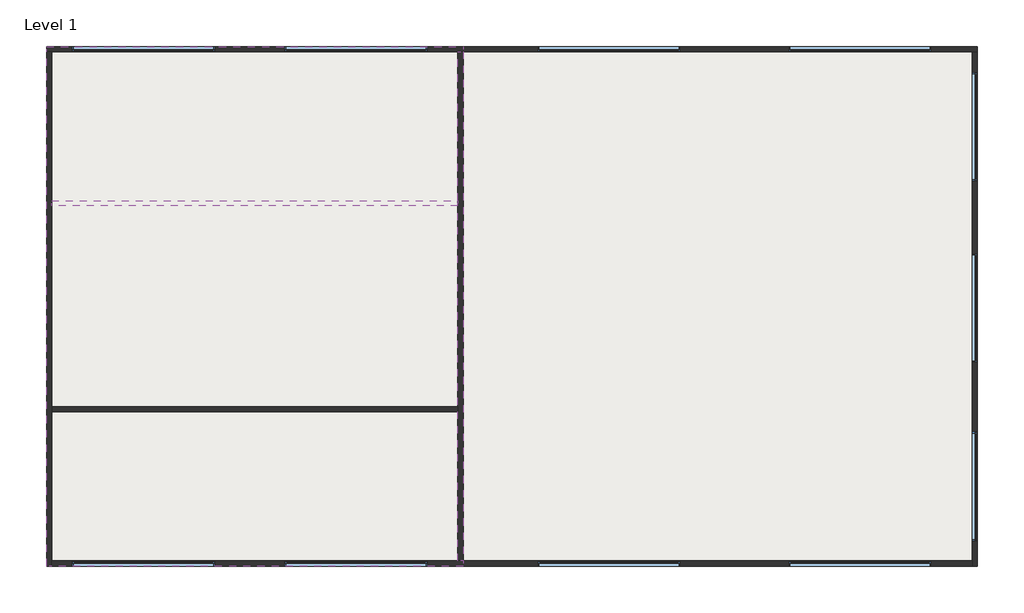
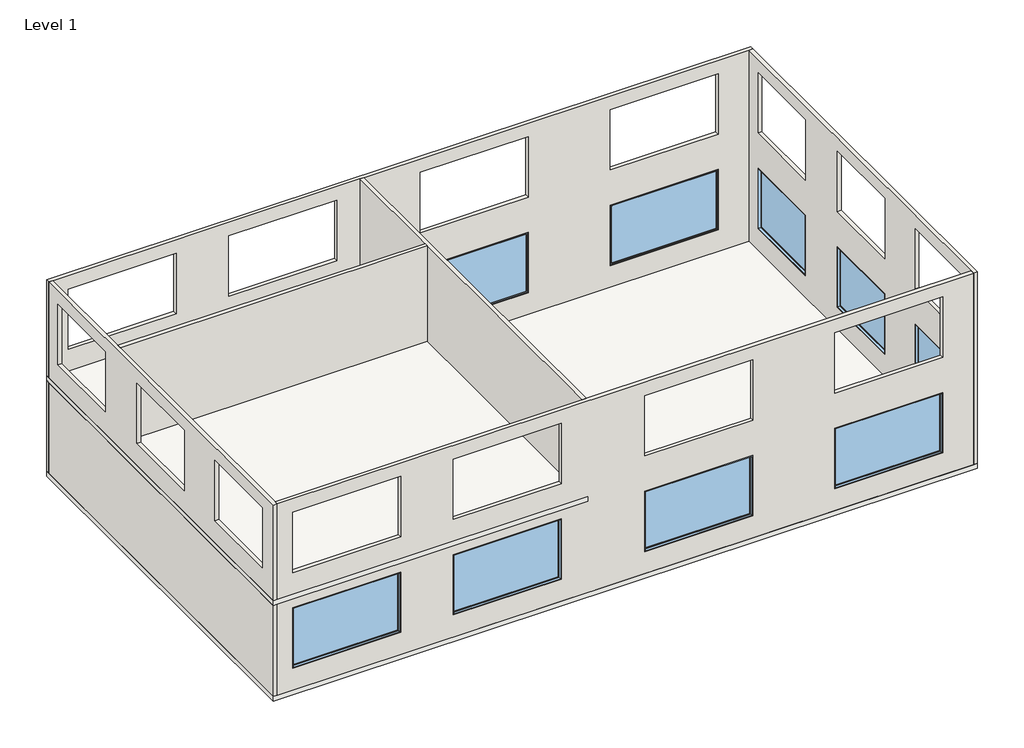
# One storey: 11 windows, 8 walls, 2 slabs.
"""IFC4 building model written with IfcOpenShell, lengths in millimetres."""

import ifcopenshell
import ifcopenshell.guid

model = None  # the IFC model being written
_history = None  # IfcOwnerHistory: only IFC2X3 demands one
_inside = {}  # id of a spatial element -> (the spatial element, [elements in it])
_under = {}  # id of a project, library or spatial element -> (it, [spatial elements below it])
_declared = {}  # id of a project -> (the project, [libraries it declares])
_typed = {}  # id of a type object -> (the type object, [elements of that type])
_made_of = {}  # id of a material, layer set ... -> (it, [elements and type objects made of it])


def new_model(schema):
    """Start an empty IFC model of exactly this schema.

    Asked for "IFC4X3", IfcOpenShell would pick the latest addendum, in which some entities
    have other attributes; the version numbers below select the first issue.
    IFC2X3 requires an IfcOwnerHistory on every rooted entity: one is made here for all.
    """
    global model, _history
    if schema == "IFC4X3":
        model = ifcopenshell.file(schema_version=(4, 3, 0, 0))
    else:
        model = ifcopenshell.file(schema=schema)
    _inside.clear()
    _under.clear()
    _declared.clear()
    _typed.clear()
    _made_of.clear()
    _history = None
    if model.schema == "IFC2X3":
        org = make("IfcOrganization", Name="unknown")
        user = make(
            "IfcPersonAndOrganization",
            ThePerson=make("IfcPerson", FamilyName="unknown"),
            TheOrganization=org,
        )
        app = make(
            "IfcApplication",
            ApplicationDeveloper=org,
            Version="unknown",
            ApplicationFullName="unknown",
            ApplicationIdentifier="unknown",
        )
        _history = make(
            "IfcOwnerHistory",
            OwningUser=user,
            OwningApplication=app,
            ChangeAction="ADDED",
            CreationDate=0,
        )
    return model


def make(cls, **values):
    """One entity of the class cls with the attributes given. An attribute that is None is left unset."""
    return model.create_entity(
        cls, **{name: value for name, value in values.items() if value is not None}
    )


def rooted(cls, **values):
    """An entity with a GlobalId (a new one), such as an element, a storey or a relation."""
    return make(cls, GlobalId=ifcopenshell.guid.new(), OwnerHistory=_history, **values)


def si_unit(unit_type, name, prefix=None):
    """IfcSIUnit, for example si_unit("LENGTHUNIT", "METRE", prefix="MILLI")."""
    return make("IfcSIUnit", UnitType=unit_type, Prefix=prefix, Name=name)


def assignment(units):
    """IfcUnitAssignment: the units of a project."""
    return None if units is None else make("IfcUnitAssignment", Units=units)


def point(xyz):
    """IfcCartesianPoint."""
    return None if xyz is None else make("IfcCartesianPoint", Coordinates=xyz)


def direction(xyz):
    """IfcDirection."""
    return None if xyz is None else make("IfcDirection", DirectionRatios=xyz)


def frame(location, z_axis=None, x_axis=None):
    """IfcAxis2Placement3D, a coordinate frame: its origin and axes. An axis left out is left unset."""
    return make(
        "IfcAxis2Placement3D",
        Location=point(location),
        Axis=direction(z_axis),
        RefDirection=direction(x_axis),
    )


def origin():
    """The frame at (0, 0, 0) with its axes left unset."""
    return frame((0.0, 0.0, 0.0))


def origin_with_axes():
    """The frame at (0, 0, 0) with the z axis (0, 0, 1) and the x axis (1, 0, 0) written out."""
    return frame((0.0, 0.0, 0.0), z_axis=(0.0, 0.0, 1.0), x_axis=(1.0, 0.0, 0.0))


def place(relative_to, where):
    """IfcLocalPlacement: puts the frame where relative to a parent placement (None: the world)."""
    return make(
        "IfcLocalPlacement", PlacementRelTo=relative_to, RelativePlacement=where
    )


def context(
    kind, dimensions, precision=None, world=None, true_north=None, identifier=None
):
    """IfcGeometricRepresentationContext, for example the 3D "Model" context."""
    return make(
        "IfcGeometricRepresentationContext",
        ContextIdentifier=identifier,
        ContextType=kind,
        CoordinateSpaceDimension=dimensions,
        Precision=precision,
        WorldCoordinateSystem=world,
        TrueNorth=true_north,
    )


def project(units=None, contexts=None):
    """IfcProject with its units and contexts."""
    return rooted(
        "IfcProject",
        Name="project",
        RepresentationContexts=contexts,
        UnitsInContext=assignment(units),
    )


def spatial(cls, under=None, at=None, **own):
    """A site, building, storey or space (cls), placed at a placement, below another one or the project."""
    s = rooted(cls, ObjectPlacement=at, **own)
    if under is not None:
        _under.setdefault(under.id(), (under, []))[1].append(s)
    return s


def polyline(points):
    """IfcPolyline through the points."""
    return make("IfcPolyline", Points=[point(p) for p in points])


def outline(outer, holes=None, kind="AREA"):
    """IfcArbitraryClosedProfileDef: a profile drawn as a closed curve; with holes, ...WithVoids."""
    if holes is None:
        return make("IfcArbitraryClosedProfileDef", ProfileType=kind, OuterCurve=outer)
    return make(
        "IfcArbitraryProfileDefWithVoids",
        ProfileType=kind,
        OuterCurve=outer,
        InnerCurves=holes,
    )


def extrude(swept, where, along, depth):
    """IfcExtrudedAreaSolid: the profile swept, set in the frame where, extruded along a direction by depth."""
    return make(
        "IfcExtrudedAreaSolid",
        SweptArea=swept,
        Position=where,
        ExtrudedDirection=direction(along),
        Depth=depth,
    )


def faces_of(points, faces, orient=None, outer=None):
    """IfcFace entities. A face is a list of loops; a loop is a list of indices into points, from 0.

    orient and outer hold one flag for each loop. By default every Orientation is true, the
    first loop of a face is its IfcFaceOuterBound and the others are IfcFaceBound.
    """
    made = []
    for i, loops in enumerate(faces):
        bounds = []
        for j, loop in enumerate(loops):
            is_outer = j == 0 if outer is None else outer[i][j]
            bounds.append(
                make(
                    "IfcFaceOuterBound" if is_outer else "IfcFaceBound",
                    Bound=make("IfcPolyLoop", Polygon=[points[k] for k in loop]),
                    Orientation=True if orient is None else orient[i][j],
                )
            )
        made.append(make("IfcFace", Bounds=bounds))
    return made


def faceted_brep(points, faces, orient=None, outer=None, voids=None):
    """IfcFacetedBrep: a solid bounded by flat faces; with voids (closed shells), ...WithVoids."""
    shared = [point(p) for p in points]
    hull = make("IfcClosedShell", CfsFaces=faces_of(shared, faces, orient, outer))
    if voids is None:
        return make("IfcFacetedBrep", Outer=hull)
    return make(
        "IfcFacetedBrepWithVoids",
        Outer=hull,
        Voids=[
            make(cls, CfsFaces=faces_of(shared, fs, o, b)) for cls, fs, o, b in voids
        ],
    )


def shape(context_of_items, identifier, shape_type, items):
    """IfcShapeRepresentation: the items that make up one representation, for example the "Body"."""
    return make(
        "IfcShapeRepresentation",
        ContextOfItems=context_of_items,
        RepresentationIdentifier=identifier,
        RepresentationType=shape_type,
        Items=items,
    )


def source(mapping_origin, context_of_items, identifier, shape_type, items):
    """IfcRepresentationMap: a shape defined once, which mapped items show again and again."""
    return make(
        "IfcRepresentationMap",
        MappingOrigin=mapping_origin,
        MappedRepresentation=shape(context_of_items, identifier, shape_type, items),
    )


def transform(
    local_origin,
    x_axis=None,
    y_axis=None,
    z_axis=None,
    scale=None,
    scale2=None,
    scale3=None,
    uniform=True,
):
    """IfcCartesianTransformationOperator3D, or its non-uniform kind. x_axis, y_axis, z_axis: its Axis1, 2, 3."""
    if uniform:
        return make(
            "IfcCartesianTransformationOperator3D",
            Axis1=direction(x_axis),
            Axis2=direction(y_axis),
            LocalOrigin=point(local_origin),
            Scale=scale,
            Axis3=direction(z_axis),
        )
    return make(
        "IfcCartesianTransformationOperator3DnonUniform",
        Axis1=direction(x_axis),
        Axis2=direction(y_axis),
        LocalOrigin=point(local_origin),
        Scale=scale,
        Axis3=direction(z_axis),
        Scale2=scale2,
        Scale3=scale3,
    )


def mapped(mapping_source, mapping_target):
    """IfcMappedItem: shows the shape of a source again, moved by a transform."""
    return make(
        "IfcMappedItem", MappingSource=mapping_source, MappingTarget=mapping_target
    )


def made_of(thing, what):
    """Note that an element or type object is made of a material, layer set ...; save() writes the relation."""
    if what is not None:
        _made_of.setdefault(what.id(), (what, []))[1].append(thing)
    return thing


def element(
    cls,
    number,
    at=None,
    inside=None,
    cuts=None,
    type_object=None,
    material=None,
    context=None,
    identifier="Body",
    shape_type=None,
    held_by="IfcProductDefinitionShape",
    body=None,
    shapes=None,
    **own,
):
    """One element of the class cls, such as IfcWall. Its Tag is "e" and its number.

    at: its placement. inside: the storey or other place that contains it. cuts: it is an
    opening in that element (IfcRelVoidsElement). A single representation is given by context,
    identifier, shape_type and body (its items); several are given by shapes. held_by: the class
    of the entity that holds the representations. save() writes the other relations.
    """
    e = rooted(cls, Tag="e%d" % number, ObjectPlacement=at, **own)
    if body is not None:
        shapes = [shape(context, identifier, shape_type, body)]
    if shapes is not None:
        e.Representation = make(held_by, Representations=shapes)
    if inside is not None:
        _inside.setdefault(inside.id(), (inside, []))[1].append(e)
    if cuts is not None:
        rooted(
            "IfcRelVoidsElement", RelatingBuildingElement=cuts, RelatedOpeningElement=e
        )
    if type_object is not None:
        _typed.setdefault(type_object.id(), (type_object, []))[1].append(e)
    return made_of(e, material)


def aggregate(whole, parts):
    """IfcRelAggregates: a whole, such as a stair, and the parts it consists of."""
    return rooted("IfcRelAggregates", RelatingObject=whole, RelatedObjects=parts)


def save(model, path):
    """Write the relations noted so far, then the file.

    IfcRelAggregates (storeys below a building ...), IfcRelContainedInSpatialStructure (elements
    in a storey), IfcRelDefinesByType, IfcRelAssociatesMaterial and IfcRelDeclares: one each for
    every whole, place, type object, material and project.
    """
    for whole, parts in _under.values():
        aggregate(whole, parts)
    for where, things in _inside.values():
        rooted(
            "IfcRelContainedInSpatialStructure",
            RelatedElements=things,
            RelatingStructure=where,
        )
    for kind, things in _typed.values():
        rooted("IfcRelDefinesByType", RelatedObjects=things, RelatingType=kind)
    for what, things in _made_of.values():
        rooted("IfcRelAssociatesMaterial", RelatedObjects=things, RelatingMaterial=what)
    for by, libraries in _declared.values():
        rooted("IfcRelDeclares", RelatingContext=by, RelatedDefinitions=libraries)
    model.write(path)


def m_fixed_2500x_4228mm_fd5e51e7(model_context):
    return source(origin(), model_context, "Body", "SweptSolid", [
        extrude(outline(polyline([(-2050.8, 54.2), (2050.8, 54.2), (2050.8, 42.2), (-2050.8, 42.2), (-2050.8, 54.2)])), frame((0.0, 0.0, 368.0), z_axis=(0.0, 0.0, 1.0), x_axis=(1.0, 0.0, 0.0)), (0.0, 0.0, 1.0), 2374.0),
        extrude(outline(polyline([(2786.0, -2094.8), (324.0, -2094.8), (324.0, 2094.8), (2786.0, 2094.8), (2786.0, -2094.8)]), holes=[polyline([(2742.0, -2050.8), (2742.0, 2050.8), (368.0, 2050.8), (368.0, -2050.8), (2742.0, -2050.8)])]), frame((0.0, 26.2, 0.0), z_axis=(0.0, 1.0, 0.0), x_axis=(0.0, 0.0, 1.0)), (0.0, 0.0, 1.0), 44.0),
        extrude(outline(polyline([(2805.0, -2113.8), (305.0, -2113.8), (305.0, 2113.8), (2805.0, 2113.8), (2805.0, -2113.8)]), holes=[polyline([(2786.0, -2094.8), (2786.0, 2094.8), (324.0, 2094.8), (324.0, -2094.8), (2786.0, -2094.8)])]), frame((0.0, 26.2, 0.0), z_axis=(0.0, 1.0, 0.0), x_axis=(0.0, 0.0, 1.0)), (0.0, 0.0, 1.0), 63.0),
        extrude(outline(polyline([(2805.0, -2113.8), (305.0, -2113.8), (305.0, 2113.8), (2805.0, 2113.8), (2805.0, -2113.8)]), holes=[polyline([(2773.0, -2081.8), (2773.0, 2081.8), (337.0, 2081.8), (337.0, -2081.8), (2773.0, -2081.8)])]), frame((0.0, -63.2, 0.0), z_axis=(0.0, 1.0, 0.0), x_axis=(0.0, 0.0, 1.0)), (0.0, 0.0, 1.0), 89.4),
    ])


def m_fixed_2500x_4228mm_f14c179f(model_context):
    return source(origin(), model_context, "Body", "SweptSolid", [
        extrude(outline(polyline([(-2050.8, -54.2), (-2050.8, -42.2), (2050.8, -42.2), (2050.8, -54.2), (-2050.8, -54.2)])), frame((0.0, 0.0, 368.0), z_axis=(0.0, 0.0, 1.0), x_axis=(1.0, 0.0, 0.0)), (0.0, 0.0, 1.0), 2374.0),
        extrude(outline(polyline([(2786.0, -2094.8), (324.0, -2094.8), (324.0, 2094.8), (2786.0, 2094.8), (2786.0, -2094.8)]), holes=[polyline([(2742.0, -2050.8), (2742.0, 2050.8), (368.0, 2050.8), (368.0, -2050.8), (2742.0, -2050.8)])]), frame((0.0, -70.2, 0.0), z_axis=(0.0, 1.0, 0.0), x_axis=(0.0, 0.0, 1.0)), (0.0, 0.0, 1.0), 44.0),
        extrude(outline(polyline([(2805.0, -2113.8), (305.0, -2113.8), (305.0, 2113.8), (2805.0, 2113.8), (2805.0, -2113.8)]), holes=[polyline([(2786.0, -2094.8), (2786.0, 2094.8), (324.0, 2094.8), (324.0, -2094.8), (2786.0, -2094.8)])]), frame((0.0, -89.2, 0.0), z_axis=(0.0, 1.0, 0.0), x_axis=(0.0, 0.0, 1.0)), (0.0, 0.0, 1.0), 63.0),
        extrude(outline(polyline([(2805.0, -2113.8), (305.0, -2113.8), (305.0, 2113.8), (2805.0, 2113.8), (2805.0, -2113.8)]), holes=[polyline([(2773.0, -2081.8), (2773.0, 2081.8), (337.0, 2081.8), (337.0, -2081.8), (2773.0, -2081.8)])]), frame((0.0, -26.2, 0.0), z_axis=(0.0, 1.0, 0.0), x_axis=(0.0, 0.0, 1.0)), (0.0, 0.0, 1.0), 89.4),
    ])


def m_fixed_2500x_3220mm_8b997f8c(model_context):
    return source(origin(), model_context, "Body", "SweptSolid", [
        extrude(outline(polyline([(-1546.8, -54.2), (-1546.8, -42.2), (1546.8, -42.2), (1546.8, -54.2), (-1546.8, -54.2)])), frame((0.0, 0.0, 368.0), z_axis=(0.0, 0.0, 1.0), x_axis=(1.0, 0.0, 0.0)), (0.0, 0.0, 1.0), 2374.0),
        extrude(outline(polyline([(2786.0, -1590.8), (324.0, -1590.8), (324.0, 1590.8), (2786.0, 1590.8), (2786.0, -1590.8)]), holes=[polyline([(2742.0, -1546.8), (2742.0, 1546.8), (368.0, 1546.8), (368.0, -1546.8), (2742.0, -1546.8)])]), frame((0.0, -70.2, 0.0), z_axis=(0.0, 1.0, 0.0), x_axis=(0.0, 0.0, 1.0)), (0.0, 0.0, 1.0), 44.0),
        extrude(outline(polyline([(2805.0, -1609.8), (305.0, -1609.8), (305.0, 1609.8), (2805.0, 1609.8), (2805.0, -1609.8)]), holes=[polyline([(2786.0, -1590.8), (2786.0, 1590.8), (324.0, 1590.8), (324.0, -1590.8), (2786.0, -1590.8)])]), frame((0.0, -89.2, 0.0), z_axis=(0.0, 1.0, 0.0), x_axis=(0.0, 0.0, 1.0)), (0.0, 0.0, 1.0), 63.0),
        extrude(outline(polyline([(2805.0, -1609.8), (305.0, -1609.8), (305.0, 1609.8), (2805.0, 1609.8), (2805.0, -1609.8)]), holes=[polyline([(2773.0, -1577.8), (2773.0, 1577.8), (337.0, 1577.8), (337.0, -1577.8), (2773.0, -1577.8)])]), frame((0.0, -26.2, 0.0), z_axis=(0.0, 1.0, 0.0), x_axis=(0.0, 0.0, 1.0)), (0.0, 0.0, 1.0), 89.4),
    ])


model = new_model("IFC4")

# Units and contexts
model_context = context("Model", 3, world=origin())
ifc_project = project(units=[si_unit("LENGTHUNIT", "METRE", prefix="MILLI")], contexts=[model_context])

# Site, building, storey
site = spatial("IfcSite", under=ifc_project)
building = spatial("IfcBuilding", under=site)
storey = spatial("IfcBuildingStorey", under=building, Name="Level 1", Elevation=0.0)

# Slabs
placement = place(None, origin())
element("IfcSlab", 1, ObjectType="160mm Concrete With 50mm Metal Deck", at=placement, inside=storey, context=model_context, shape_type="Brep", body=[
    faceted_brep([(29068.464681, 11296.9802217, -210.0), (29068.464681, -4095.4197783, -210.0), (1484.064681, -4095.4197783, -210.0), (1484.064681, 11296.9802217, -210.0), (29068.464681, 11296.9802217, 0.0), (1484.064681, 11296.9802217, 0.0), (1484.064681, -4095.4197783, 0.0), (28916.064681, -4095.4197783, 0.0), (29068.464681, -4095.4197783, 0.0), (29068.464681, 11144.5802217, 0.0)], [[[0, 1, 2, 3]], [[4, 5, 6, 7, 8, 9]], [[1, 0, 4, 9, 8]], [[2, 1, 8, 7, 6]], [[3, 2, 6, 5]], [[0, 3, 5, 4]]]),
])
element("IfcSlab", 2, ObjectType="160mm Concrete With 50mm Metal Deck", at=placement, inside=storey, context=model_context, shape_type="Brep", body=[
    faceted_brep([(13828.464681, 11296.9802217, 3752.4), (13828.464681, 11144.5802217, 3752.4), (13828.464681, -3943.0197783, 3752.4), (13828.464681, -4095.4197783, 3752.4), (1636.464681, -4095.4197783, 3752.4), (1484.064681, -4095.4197783, 3752.4), (1484.064681, 11144.5802217, 3752.4), (1484.064681, 11296.9802217, 3752.4), (13828.464681, 11296.9802217, 3962.4), (1484.064681, 11296.9802217, 3962.4), (1484.064681, 11144.5802217, 3962.4), (1484.064681, -4095.4197783, 3962.4), (1636.464681, -4095.4197783, 3962.4), (13828.464681, -4095.4197783, 3962.4), (13828.464681, -3943.0197783, 3962.4), (13828.464681, 11144.5802217, 3962.4)], [[[0, 1, 2, 3, 4, 5, 6, 7]], [[8, 9, 10, 11, 12, 13, 14, 15]], [[3, 2, 1, 0, 8, 15, 14, 13]], [[5, 4, 3, 13, 12, 11]], [[7, 6, 5, 11, 10, 9]], [[0, 7, 9, 8]]]),
])

# Walls
element("IfcWall", 3, ObjectType="Generic - 152.4mm", at=placement, inside=storey, context=model_context, shape_type="Brep", body=[
    faceted_brep([(1484.064681, 11144.5802217, 0.0), (1636.464681, 11144.5802217, 0.0), (13676.064681, 11144.5802217, 0.0), (13828.464681, 11144.5802217, 0.0), (28916.064681, 11144.5802217, 0.0), (29068.464681, 11144.5802217, 0.0), (29068.464681, 11144.5802217, 7924.8), (28916.064681, 11144.5802217, 7924.8), (13828.464681, 11144.5802217, 7924.8), (13676.064681, 11144.5802217, 7924.8), (1636.464681, 11144.5802217, 7924.8), (1484.064681, 11144.5802217, 7924.8), (1484.064681, 11144.5802217, 3962.4), (13676.064681, 11144.5802217, 3962.4), (13828.464681, 11144.5802217, 3962.4), (13828.464681, 11144.5802217, 3752.4), (13676.064681, 11144.5802217, 3752.4), (1484.064681, 11144.5802217, 3752.4), (6474.064681, 11144.5802217, 3402.4), (6474.064681, 11144.5802217, 902.4), (2246.464681, 11144.5802217, 902.4), (2246.464681, 11144.5802217, 3402.4), (12766.064681, 11144.5802217, 3402.4), (12766.064681, 11144.5802217, 902.4), (8538.464681, 11144.5802217, 902.4), (8538.464681, 11144.5802217, 3402.4), (20266.064681, 11144.5802217, 3402.4), (20266.064681, 11144.5802217, 902.4), (16038.464681, 11144.5802217, 902.4), (16038.464681, 11144.5802217, 3402.4), (27706.064681, 11144.5802217, 3402.4), (27706.064681, 11144.5802217, 902.4), (23478.464681, 11144.5802217, 902.4), (23478.464681, 11144.5802217, 3402.4), (27706.064681, 11144.5802217, 7362.4), (27706.064681, 11144.5802217, 4862.4), (23478.464681, 11144.5802217, 4862.4), (23478.464681, 11144.5802217, 7362.4), (20266.064681, 11144.5802217, 7362.4), (20266.064681, 11144.5802217, 4862.4), (16038.464681, 11144.5802217, 4862.4), (16038.464681, 11144.5802217, 7362.4), (12766.064681, 11144.5802217, 7362.4), (12766.064681, 11144.5802217, 4862.4), (8538.464681, 11144.5802217, 4862.4), (8538.464681, 11144.5802217, 7362.4), (6474.064681, 11144.5802217, 7362.4), (6474.064681, 11144.5802217, 4862.4), (2246.464681, 11144.5802217, 4862.4), (2246.464681, 11144.5802217, 7362.4), (29068.464681, 11296.9802217, 0.0), (1484.064681, 11296.9802217, 0.0), (1484.064681, 11296.9802217, 3752.4), (13828.464681, 11296.9802217, 3752.4), (13828.464681, 11296.9802217, 3962.4), (1484.064681, 11296.9802217, 3962.4), (1484.064681, 11296.9802217, 7924.8), (29068.464681, 11296.9802217, 7924.8), (6474.064681, 11296.9802217, 902.4), (6474.064681, 11296.9802217, 3402.4), (2246.464681, 11296.9802217, 3402.4), (2246.464681, 11296.9802217, 902.4), (12766.064681, 11296.9802217, 902.4), (12766.064681, 11296.9802217, 3402.4), (8538.464681, 11296.9802217, 3402.4), (8538.464681, 11296.9802217, 902.4), (20266.064681, 11296.9802217, 902.4), (20266.064681, 11296.9802217, 3402.4), (16038.464681, 11296.9802217, 3402.4), (16038.464681, 11296.9802217, 902.4), (27706.064681, 11296.9802217, 902.4), (27706.064681, 11296.9802217, 3402.4), (23478.464681, 11296.9802217, 3402.4), (23478.464681, 11296.9802217, 902.4), (27706.064681, 11296.9802217, 4862.4), (27706.064681, 11296.9802217, 7362.4), (23478.464681, 11296.9802217, 7362.4), (23478.464681, 11296.9802217, 4862.4), (20266.064681, 11296.9802217, 4862.4), (20266.064681, 11296.9802217, 7362.4), (16038.464681, 11296.9802217, 7362.4), (16038.464681, 11296.9802217, 4862.4), (12766.064681, 11296.9802217, 4862.4), (12766.064681, 11296.9802217, 7362.4), (8538.464681, 11296.9802217, 7362.4), (8538.464681, 11296.9802217, 4862.4), (6474.064681, 11296.9802217, 4862.4), (6474.064681, 11296.9802217, 7362.4), (2246.464681, 11296.9802217, 7362.4), (2246.464681, 11296.9802217, 4862.4)], [[[0, 1, 2, 3, 4, 5, 6, 7, 8, 9, 10, 11, 12, 13, 14, 15, 16, 17], [18, 19, 20, 21], [22, 23, 24, 25], [26, 27, 28, 29], [30, 31, 32, 33], [34, 35, 36, 37], [38, 39, 40, 41], [42, 43, 44, 45], [46, 47, 48, 49]], [[50, 51, 52, 53, 54, 55, 56, 57], [58, 59, 60, 61], [62, 63, 64, 65], [66, 67, 68, 69], [70, 71, 72, 73], [74, 75, 76, 77], [78, 79, 80, 81], [82, 83, 84, 85], [86, 87, 88, 89]], [[5, 4, 3, 2, 1, 0, 51, 50]], [[11, 10, 9, 8, 7, 6, 57, 56]], [[6, 5, 50, 57]], [[11, 56, 55, 12]], [[51, 0, 17, 52]], [[59, 58, 19, 18]], [[60, 59, 18, 21]], [[61, 60, 21, 20]], [[58, 61, 20, 19]], [[63, 62, 23, 22]], [[64, 63, 22, 25]], [[65, 64, 25, 24]], [[62, 65, 24, 23]], [[67, 66, 27, 26]], [[68, 67, 26, 29]], [[69, 68, 29, 28]], [[66, 69, 28, 27]], [[71, 70, 31, 30]], [[72, 71, 30, 33]], [[73, 72, 33, 32]], [[70, 73, 32, 31]], [[75, 74, 35, 34]], [[76, 75, 34, 37]], [[77, 76, 37, 36]], [[74, 77, 36, 35]], [[79, 78, 39, 38]], [[80, 79, 38, 41]], [[81, 80, 41, 40]], [[78, 81, 40, 39]], [[83, 82, 43, 42]], [[84, 83, 42, 45]], [[85, 84, 45, 44]], [[82, 85, 44, 43]], [[87, 86, 47, 46]], [[88, 87, 46, 49]], [[89, 88, 49, 48]], [[86, 89, 48, 47]], [[15, 53, 52, 17, 16]], [[54, 14, 13, 12, 55]], [[53, 15, 14, 54]]]),
])
element("IfcWall", 4, ObjectType="Generic - 152.4mm", at=placement, inside=storey, context=model_context, shape_type="Brep", body=[
    faceted_brep([(28916.064681, 11144.5802217, 0.0), (28916.064681, -3943.0197783, 0.0), (28916.064681, -4095.4197783, 0.0), (28916.064681, -4095.4197783, 7924.8), (28916.064681, -3943.0197783, 7924.8), (28916.064681, 11144.5802217, 7924.8), (28916.064681, -3343.0197783, 902.4), (28916.064681, -123.4197783, 902.4), (28916.064681, -123.4197783, 3402.4), (28916.064681, -3343.0197783, 3402.4), (28916.064681, 1942.9802217, 902.4), (28916.064681, 5162.5802217, 902.4), (28916.064681, 5162.5802217, 3402.4), (28916.064681, 1942.9802217, 3402.4), (28916.064681, 7310.9802217, 902.4), (28916.064681, 10530.5802217, 902.4), (28916.064681, 10530.5802217, 3402.4), (28916.064681, 7310.9802217, 3402.4), (28916.064681, -3343.0197783, 4864.8), (28916.064681, -123.4197783, 4864.8), (28916.064681, -123.4197783, 7364.8), (28916.064681, -3343.0197783, 7364.8), (28916.064681, 1942.9802217, 4864.8), (28916.064681, 5162.5802217, 4864.8), (28916.064681, 5162.5802217, 7364.8), (28916.064681, 1942.9802217, 7364.8), (28916.064681, 7310.9802217, 4864.8), (28916.064681, 10530.5802217, 4864.8), (28916.064681, 10530.5802217, 7364.8), (28916.064681, 7310.9802217, 7364.8), (29068.464681, 11144.5802217, 0.0), (29068.464681, 11144.5802217, 7924.8), (29068.464681, -4095.4197783, 7924.8), (29068.464681, -4095.4197783, 0.0), (29068.464681, -3343.0197783, 902.4), (29068.464681, -3343.0197783, 3402.4), (29068.464681, -123.4197783, 3402.4), (29068.464681, -123.4197783, 902.4), (29068.464681, 1942.9802217, 902.4), (29068.464681, 1942.9802217, 3402.4), (29068.464681, 5162.5802217, 3402.4), (29068.464681, 5162.5802217, 902.4), (29068.464681, 7310.9802217, 902.4), (29068.464681, 7310.9802217, 3402.4), (29068.464681, 10530.5802217, 3402.4), (29068.464681, 10530.5802217, 902.4), (29068.464681, -3343.0197783, 4864.8), (29068.464681, -3343.0197783, 7364.8), (29068.464681, -123.4197783, 7364.8), (29068.464681, -123.4197783, 4864.8), (29068.464681, 1942.9802217, 4864.8), (29068.464681, 1942.9802217, 7364.8), (29068.464681, 5162.5802217, 7364.8), (29068.464681, 5162.5802217, 4864.8), (29068.464681, 7310.9802217, 4864.8), (29068.464681, 7310.9802217, 7364.8), (29068.464681, 10530.5802217, 7364.8), (29068.464681, 10530.5802217, 4864.8)], [[[0, 1, 2, 3, 4, 5], [6, 7, 8, 9], [10, 11, 12, 13], [14, 15, 16, 17], [18, 19, 20, 21], [22, 23, 24, 25], [26, 27, 28, 29]], [[30, 31, 32, 33], [34, 35, 36, 37], [38, 39, 40, 41], [42, 43, 44, 45], [46, 47, 48, 49], [50, 51, 52, 53], [54, 55, 56, 57]], [[2, 1, 0, 30, 33]], [[5, 4, 3, 32, 31]], [[0, 5, 31, 30]], [[35, 34, 6, 9]], [[36, 35, 9, 8]], [[37, 36, 8, 7]], [[34, 37, 7, 6]], [[39, 38, 10, 13]], [[40, 39, 13, 12]], [[41, 40, 12, 11]], [[38, 41, 11, 10]], [[43, 42, 14, 17]], [[44, 43, 17, 16]], [[45, 44, 16, 15]], [[42, 45, 15, 14]], [[3, 2, 33, 32]], [[47, 46, 18, 21]], [[48, 47, 21, 20]], [[49, 48, 20, 19]], [[46, 49, 19, 18]], [[51, 50, 22, 25]], [[52, 51, 25, 24]], [[53, 52, 24, 23]], [[50, 53, 23, 22]], [[55, 54, 26, 29]], [[56, 55, 29, 28]], [[57, 56, 28, 27]], [[54, 57, 27, 26]]]),
])
element("IfcWall", 5, ObjectType="Generic - 152.4mm", at=placement, inside=storey, context=model_context, shape_type="Brep", body=[
    faceted_brep([(28916.064681, -3943.0197783, 0.0), (13828.464681, -3943.0197783, 0.0), (13676.064681, -3943.0197783, 0.0), (1636.464681, -3943.0197783, 0.0), (1636.464681, -3943.0197783, 3752.4), (13676.064681, -3943.0197783, 3752.4), (13828.464681, -3943.0197783, 3752.4), (13828.464681, -3943.0197783, 3962.4), (13676.064681, -3943.0197783, 3962.4), (1636.464681, -3943.0197783, 3962.4), (1636.464681, -3943.0197783, 7924.8), (13676.064681, -3943.0197783, 7924.8), (13828.464681, -3943.0197783, 7924.8), (28916.064681, -3943.0197783, 7924.8), (27706.064681, -3943.0197783, 902.4), (27706.064681, -3943.0197783, 3402.4), (23478.464681, -3943.0197783, 3402.4), (23478.464681, -3943.0197783, 902.4), (20266.064681, -3943.0197783, 902.4), (20266.064681, -3943.0197783, 3402.4), (16038.464681, -3943.0197783, 3402.4), (16038.464681, -3943.0197783, 902.4), (12766.064681, -3943.0197783, 902.4), (12766.064681, -3943.0197783, 3402.4), (8538.464681, -3943.0197783, 3402.4), (8538.464681, -3943.0197783, 902.4), (6474.064681, -3943.0197783, 902.4), (6474.064681, -3943.0197783, 3402.4), (2246.464681, -3943.0197783, 3402.4), (2246.464681, -3943.0197783, 902.4), (27706.064681, -3943.0197783, 4862.4), (27706.064681, -3943.0197783, 7362.4), (23478.464681, -3943.0197783, 7362.4), (23478.464681, -3943.0197783, 4862.4), (20266.064681, -3943.0197783, 4862.4), (20266.064681, -3943.0197783, 7362.4), (16038.464681, -3943.0197783, 7362.4), (16038.464681, -3943.0197783, 4862.4), (12766.064681, -3943.0197783, 4862.4), (12766.064681, -3943.0197783, 7362.4), (8538.464681, -3943.0197783, 7362.4), (8538.464681, -3943.0197783, 4862.4), (6474.064681, -3943.0197783, 4862.4), (6474.064681, -3943.0197783, 7362.4), (2246.464681, -3943.0197783, 7362.4), (2246.464681, -3943.0197783, 4862.4), (1636.464681, -4095.4197783, 0.0), (28916.064681, -4095.4197783, 0.0), (28916.064681, -4095.4197783, 7924.8), (1636.464681, -4095.4197783, 7924.8), (1636.464681, -4095.4197783, 3962.4), (13828.464681, -4095.4197783, 3962.4), (13828.464681, -4095.4197783, 3752.4), (1636.464681, -4095.4197783, 3752.4), (27706.064681, -4095.4197783, 3402.4), (27706.064681, -4095.4197783, 902.4), (23478.464681, -4095.4197783, 902.4), (23478.464681, -4095.4197783, 3402.4), (20266.064681, -4095.4197783, 3402.4), (20266.064681, -4095.4197783, 902.4), (16038.464681, -4095.4197783, 902.4), (16038.464681, -4095.4197783, 3402.4), (12766.064681, -4095.4197783, 3402.4), (12766.064681, -4095.4197783, 902.4), (8538.464681, -4095.4197783, 902.4), (8538.464681, -4095.4197783, 3402.4), (6474.064681, -4095.4197783, 3402.4), (6474.064681, -4095.4197783, 902.4), (2246.464681, -4095.4197783, 902.4), (2246.464681, -4095.4197783, 3402.4), (27706.064681, -4095.4197783, 7362.4), (27706.064681, -4095.4197783, 4862.4), (23478.464681, -4095.4197783, 4862.4), (23478.464681, -4095.4197783, 7362.4), (20266.064681, -4095.4197783, 7362.4), (20266.064681, -4095.4197783, 4862.4), (16038.464681, -4095.4197783, 4862.4), (16038.464681, -4095.4197783, 7362.4), (12766.064681, -4095.4197783, 7362.4), (12766.064681, -4095.4197783, 4862.4), (8538.464681, -4095.4197783, 4862.4), (8538.464681, -4095.4197783, 7362.4), (6474.064681, -4095.4197783, 7362.4), (6474.064681, -4095.4197783, 4862.4), (2246.464681, -4095.4197783, 4862.4), (2246.464681, -4095.4197783, 7362.4)], [[[0, 1, 2, 3, 4, 5, 6, 7, 8, 9, 10, 11, 12, 13], [14, 15, 16, 17], [18, 19, 20, 21], [22, 23, 24, 25], [26, 27, 28, 29], [30, 31, 32, 33], [34, 35, 36, 37], [38, 39, 40, 41], [42, 43, 44, 45]], [[46, 47, 48, 49, 50, 51, 52, 53], [54, 55, 56, 57], [58, 59, 60, 61], [62, 63, 64, 65], [66, 67, 68, 69], [70, 71, 72, 73], [74, 75, 76, 77], [78, 79, 80, 81], [82, 83, 84, 85]], [[3, 2, 1, 0, 47, 46]], [[13, 12, 11, 10, 49, 48]], [[15, 14, 55, 54]], [[16, 15, 54, 57]], [[17, 16, 57, 56]], [[14, 17, 56, 55]], [[19, 18, 59, 58]], [[20, 19, 58, 61]], [[21, 20, 61, 60]], [[18, 21, 60, 59]], [[23, 22, 63, 62]], [[24, 23, 62, 65]], [[25, 24, 65, 64]], [[22, 25, 64, 63]], [[27, 26, 67, 66]], [[28, 27, 66, 69]], [[29, 28, 69, 68]], [[26, 29, 68, 67]], [[47, 0, 13, 48]], [[3, 46, 53, 4]], [[49, 10, 9, 50]], [[31, 30, 71, 70]], [[32, 31, 70, 73]], [[33, 32, 73, 72]], [[30, 33, 72, 71]], [[35, 34, 75, 74]], [[36, 35, 74, 77]], [[37, 36, 77, 76]], [[34, 37, 76, 75]], [[39, 38, 79, 78]], [[40, 39, 78, 81]], [[41, 40, 81, 80]], [[38, 41, 80, 79]], [[43, 42, 83, 82]], [[44, 43, 82, 85]], [[45, 44, 85, 84]], [[42, 45, 84, 83]], [[52, 6, 5, 4, 53]], [[7, 51, 50, 9, 8]], [[6, 52, 51, 7]]]),
])
element("IfcWall", 6, ObjectType="Generic - 152.4mm", at=placement, inside=storey, context=model_context, shape_type="Brep", body=[
    faceted_brep([(1636.464681, -4095.4197783, 0.0), (1636.464681, -3943.0197783, 0.0), (1636.464681, 476.5802217, 0.0), (1636.464681, 628.9802217, 0.0), (1636.464681, 11144.5802217, 0.0), (1636.464681, 11144.5802217, 3752.4), (1636.464681, 628.9802217, 3752.4), (1636.464681, 476.5802217, 3752.4), (1636.464681, -3943.0197783, 3752.4), (1636.464681, -4095.4197783, 3752.4), (1484.064681, 11144.5802217, 0.0), (1484.064681, -4095.4197783, 0.0), (1484.064681, -4095.4197783, 3752.4), (1484.064681, 11144.5802217, 3752.4)], [[[0, 1, 2, 3, 4, 5, 6, 7, 8, 9]], [[10, 11, 12, 13]], [[4, 3, 2, 1, 0, 11, 10]], [[4, 10, 13, 5]], [[11, 0, 9, 12]], [[9, 8, 7, 6, 5, 13, 12]]]),
    faceted_brep([(1636.464681, 11144.5802217, 7924.8), (1636.464681, 6724.9802217, 7924.8), (1636.464681, 6572.5802217, 7924.8), (1636.464681, -3943.0197783, 7924.8), (1636.464681, -4095.4197783, 7924.8), (1636.464681, -4095.4197783, 3962.4), (1636.464681, -3943.0197783, 3962.4), (1636.464681, 6572.5802217, 3962.4), (1636.464681, 6724.9802217, 3962.4), (1636.464681, 11144.5802217, 3962.4), (1636.464681, -3343.0197783, 4864.8), (1636.464681, -3343.0197783, 7364.8), (1636.464681, -123.4197783, 7364.8), (1636.464681, -123.4197783, 4864.8), (1636.464681, 1942.9802217, 4864.8), (1636.464681, 1942.9802217, 7364.8), (1636.464681, 5162.5802217, 7364.8), (1636.464681, 5162.5802217, 4864.8), (1636.464681, 7310.9802217, 4864.8), (1636.464681, 7310.9802217, 7364.8), (1636.464681, 10530.5802217, 7364.8), (1636.464681, 10530.5802217, 4864.8), (1484.064681, -4095.4197783, 7924.8), (1484.064681, 11144.5802217, 7924.8), (1484.064681, 11144.5802217, 3962.4), (1484.064681, -4095.4197783, 3962.4), (1484.064681, -3343.0197783, 7364.8), (1484.064681, -3343.0197783, 4864.8), (1484.064681, -123.4197783, 4864.8), (1484.064681, -123.4197783, 7364.8), (1484.064681, 1942.9802217, 7364.8), (1484.064681, 1942.9802217, 4864.8), (1484.064681, 5162.5802217, 4864.8), (1484.064681, 5162.5802217, 7364.8), (1484.064681, 7310.9802217, 7364.8), (1484.064681, 7310.9802217, 4864.8), (1484.064681, 10530.5802217, 4864.8), (1484.064681, 10530.5802217, 7364.8)], [[[0, 1, 2, 3, 4, 5, 6, 7, 8, 9], [10, 11, 12, 13], [14, 15, 16, 17], [18, 19, 20, 21]], [[22, 23, 24, 25], [26, 27, 28, 29], [30, 31, 32, 33], [34, 35, 36, 37]], [[4, 3, 2, 1, 0, 23, 22]], [[23, 0, 9, 24]], [[4, 22, 25, 5]], [[11, 10, 27, 26]], [[12, 11, 26, 29]], [[13, 12, 29, 28]], [[10, 13, 28, 27]], [[15, 14, 31, 30]], [[16, 15, 30, 33]], [[17, 16, 33, 32]], [[14, 17, 32, 31]], [[19, 18, 35, 34]], [[20, 19, 34, 37]], [[21, 20, 37, 36]], [[18, 21, 36, 35]], [[9, 8, 7, 6, 5, 25, 24]]]),
])
element("IfcWall", 7, ObjectType="Generic - 152.4mm - Interior", at=placement, inside=storey, context=model_context, shape_type="Brep", body=[
    faceted_brep([(13828.464681, -3943.0197783, 0.0), (13828.464681, 11144.5802217, 0.0), (13828.464681, 11144.5802217, 3752.4), (13828.464681, -3943.0197783, 3752.4), (13676.064681, -3943.0197783, 0.0), (13676.064681, -3943.0197783, 3752.4), (13676.064681, 476.5802217, 3752.4), (13676.064681, 628.9802217, 3752.4), (13676.064681, 11144.5802217, 3752.4), (13676.064681, 11144.5802217, 0.0), (13676.064681, 628.9802217, 0.0), (13676.064681, 476.5802217, 0.0)], [[[0, 1, 2, 3]], [[4, 5, 6, 7, 8, 9, 10, 11]], [[1, 0, 4, 11, 10, 9]], [[0, 3, 5, 4]], [[2, 1, 9, 8]], [[3, 2, 8, 7, 6, 5]]]),
])
element("IfcWall", 8, ObjectType="Generic - 152.4mm - Interior", at=placement, inside=storey, context=model_context, shape_type="SweptSolid", body=[
    extrude(outline(polyline([(1636.464681, 628.9802217), (13676.064681, 628.9802217), (13676.064681, 476.5802217), (1636.464681, 476.5802217), (1636.464681, 628.9802217)])), origin_with_axes(), (0.0, 0.0, 1.0), 3752.4),
])
element("IfcWall", 9, ObjectType="Generic - 152.4mm - Interior", at=placement, inside=storey, context=model_context, shape_type="Brep", body=[
    faceted_brep([(13676.064681, 11144.5802217, 3962.4), (13676.064681, 6724.9802217, 3962.4), (13676.064681, 6572.5802217, 3962.4), (13676.064681, -3943.0197783, 3962.4), (13676.064681, -3943.0197783, 7924.8), (13676.064681, 6572.5802217, 7924.8), (13676.064681, 6724.9802217, 7924.8), (13676.064681, 11144.5802217, 7924.8), (13828.464681, 11144.5802217, 3962.4), (13828.464681, 11144.5802217, 7924.8), (13828.464681, -3943.0197783, 7924.8), (13828.464681, -3943.0197783, 3962.4)], [[[0, 1, 2, 3, 4, 5, 6, 7]], [[8, 9, 10, 11]], [[3, 2, 1, 0, 8, 11]], [[7, 6, 5, 4, 10, 9]], [[4, 3, 11, 10]], [[0, 7, 9, 8]]]),
])
element("IfcWall", 10, ObjectType="Generic - 152.4mm - Interior", at=placement, inside=storey, context=model_context, shape_type="SweptSolid", body=[
    extrude(outline(polyline([(1636.464681, 6724.9802217), (13676.064681, 6724.9802217), (13676.064681, 6572.5802217), (1636.464681, 6572.5802217), (1636.464681, 6724.9802217)])), frame((0.0, 0.0, 3962.4), z_axis=(0.0, 0.0, 1.0), x_axis=(1.0, 0.0, 0.0)), (0.0, 0.0, 1.0), 3962.4),
])

# Windows
m_fixed_2500x_4228mm_shape = m_fixed_2500x_4228mm_fd5e51e7(model_context)
element("IfcWindow", 11, ObjectType="M_Fixed : 2500X 4228mm", at=placement, inside=storey, context=model_context, shape_type="MappedRepresentation", body=[
    mapped(m_fixed_2500x_4228mm_shape, transform((4360.264681, 11233.7802217, 597.4), x_axis=(-1.0, 0.0, 0.0), y_axis=(0.0, -1.0, 0.0), z_axis=(0.0, 0.0, 1.0))),
])
element("IfcWindow", 12, ObjectType="M_Fixed : 2500X 4228mm", at=placement, inside=storey, context=model_context, shape_type="MappedRepresentation", body=[
    mapped(m_fixed_2500x_4228mm_shape, transform((10652.264681, 11233.7802217, 597.4), x_axis=(-1.0, 0.0, 0.0), y_axis=(0.0, -1.0, 0.0), z_axis=(0.0, 0.0, 1.0))),
])
element("IfcWindow", 13, ObjectType="M_Fixed : 2500X 4228mm", at=placement, inside=storey, context=model_context, shape_type="MappedRepresentation", body=[
    mapped(m_fixed_2500x_4228mm_shape, transform((18152.264681, 11233.7802217, 597.4), x_axis=(-1.0, 0.0, 0.0), y_axis=(0.0, -1.0, 0.0), z_axis=(0.0, 0.0, 1.0))),
])
element("IfcWindow", 14, ObjectType="M_Fixed : 2500X 4228mm", at=placement, inside=storey, context=model_context, shape_type="MappedRepresentation", body=[
    mapped(m_fixed_2500x_4228mm_shape, transform((25592.264681, 11233.7802217, 597.4), x_axis=(-1.0, 0.0, 0.0), y_axis=(0.0, -1.0, 0.0), z_axis=(0.0, 0.0, 1.0))),
])
m_fixed_2500x_4228mm_2_shape = m_fixed_2500x_4228mm_f14c179f(model_context)
element("IfcWindow", 15, ObjectType="M_Fixed : 2500X 4228mm", at=placement, inside=storey, context=model_context, shape_type="MappedRepresentation", body=[
    mapped(m_fixed_2500x_4228mm_2_shape, transform((4360.264681, -4032.2197783, 597.4), x_axis=(-1.0, 0.0, 0.0), y_axis=(0.0, -1.0, 0.0), z_axis=(0.0, 0.0, 1.0))),
])
element("IfcWindow", 16, ObjectType="M_Fixed : 2500X 4228mm", at=placement, inside=storey, context=model_context, shape_type="MappedRepresentation", body=[
    mapped(m_fixed_2500x_4228mm_2_shape, transform((10652.264681, -4032.2197783, 597.4), x_axis=(-1.0, 0.0, 0.0), y_axis=(0.0, -1.0, 0.0), z_axis=(0.0, 0.0, 1.0))),
])
element("IfcWindow", 17, ObjectType="M_Fixed : 2500X 4228mm", at=placement, inside=storey, context=model_context, shape_type="MappedRepresentation", body=[
    mapped(m_fixed_2500x_4228mm_2_shape, transform((18152.264681, -4032.2197783, 597.4), x_axis=(-1.0, 0.0, 0.0), y_axis=(0.0, -1.0, 0.0), z_axis=(0.0, 0.0, 1.0))),
])
element("IfcWindow", 18, ObjectType="M_Fixed : 2500X 4228mm", at=placement, inside=storey, context=model_context, shape_type="MappedRepresentation", body=[
    mapped(m_fixed_2500x_4228mm_2_shape, transform((25592.264681, -4032.2197783, 597.4), x_axis=(-1.0, 0.0, 0.0), y_axis=(0.0, -1.0, 0.0), z_axis=(0.0, 0.0, 1.0))),
])
m_fixed_2500x_3220mm_shape = m_fixed_2500x_3220mm_8b997f8c(model_context)
element("IfcWindow", 19, ObjectType="M_Fixed : 2500x 3220mm", at=placement, inside=storey, context=model_context, shape_type="MappedRepresentation", body=[
    mapped(m_fixed_2500x_3220mm_shape, transform((28979.264681, 8920.7802217, 597.4), x_axis=(0.0, 1.0, 0.0), y_axis=(-1.0, 0.0, 0.0), z_axis=(0.0, 0.0, 1.0))),
])
element("IfcWindow", 20, ObjectType="M_Fixed : 2500x 3220mm", at=placement, inside=storey, context=model_context, shape_type="MappedRepresentation", body=[
    mapped(m_fixed_2500x_3220mm_shape, transform((28979.264681, 3552.7802217, 597.4), x_axis=(0.0, 1.0, 0.0), y_axis=(-1.0, 0.0, 0.0), z_axis=(0.0, 0.0, 1.0))),
])
element("IfcWindow", 21, ObjectType="M_Fixed : 2500x 3220mm", at=placement, inside=storey, context=model_context, shape_type="MappedRepresentation", body=[
    mapped(m_fixed_2500x_3220mm_shape, transform((28979.264681, -1733.2197783, 597.4), x_axis=(0.0, 1.0, 0.0), y_axis=(-1.0, 0.0, 0.0), z_axis=(0.0, 0.0, 1.0))),
])

save(model, "model.ifc")

# Revit data of these elements
# Project information
#   Project Issue Date = "Issue Date"
#   Project Status = "Project Status"
#   Client Name = "Owner"
#   Project Address = "Enter address here"
#   Project Name = "Project Name"
#   Project Number = "Project Number"
# Type "160mm Concrete With 50mm Metal Deck"
#   Function = 0
#   Layers, outside or top first: 210 mm no material (function 1); 0 mm "Metal Deck" (function 200)
# Type "Generic - 152.4mm"
#   Layers, outside or top first: 152.4 mm no material (function 1)
# Type "Generic - 152.4mm - Interior"
#   Layers, outside or top first: 152.4 mm no material (function 1)
# Type "M_Fixed : 2500X 4228mm"
#   Type Mark = "25"
#   Height = 2500 mm
#   Default Sill Height = 305 mm
#   Width = 4227.6 mm
#   Window Inset = 19 mm
#   Frame Exterior Material = Sash
#   Frame Interior Material = Sash
#   Glass Pane Material = Glass
#   Sash = Sash
#   Wall Closure = (empty or 0)
# Type "M_Fixed : 2500x 3220mm"
#   Type Mark = "26"
#   Height = 2500 mm
#   Default Sill Height = 305 mm
#   Width = 3219.6 mm
#   Window Inset = 19 mm
#   Frame Exterior Material = Sash
#   Frame Interior Material = Sash
#   Glass Pane Material = Glass
#   Sash = Sash
#   Wall Closure = (empty or 0)
# Element 1 (IfcSlab, "160mm Concrete With 50mm Metal Deck")
#   Height Offset From Level = 0 mm
#   Phase Created = New Construction
#   Materials on its faces: "Metal Deck", "Default Floor"
# Element 2 (IfcSlab, "160mm Concrete With 50mm Metal Deck")
#   Height Offset From Level = 3962.4 mm
#   Phase Created = New Construction
#   Materials on its faces: "Metal Deck", "Default Floor"
# Elements 3, 4, 5, 6 (IfcWall, "Generic - 152.4mm")
#   Top Offset = 0 mm
#   Base Offset = 0 mm
#   wall height = 7924.8 mm
#   Phase Created = New Construction
#   Base Constraint = Level 1
#   Top Constraint = Roof Level
#   Materials on its faces: "Default Wall"
# Element 7 (IfcWall, "Generic - 152.4mm - Interior")
#   Top Offset = 3962.4 mm
#   Base Offset = 0 mm
#   wall height = 3752.4 mm
#   Phase Created = New Construction
#   Base Constraint = Level 1
#   Top Constraint = Level 1
#   Materials on its faces: "Default Wall"
# Element 8 (IfcWall, "Generic - 152.4mm - Interior")
#   Top Offset = 3862.4 mm
#   Base Offset = 0 mm
#   wall height = 3752.4 mm
#   Phase Created = New Construction
#   Base Constraint = Level 1
#   Top Constraint = Level 1
#   Materials on its faces: "Default Wall"
# Elements 9, 10 (IfcWall, "Generic - 152.4mm - Interior")
#   built-in parameter 1001111 = 3962.4 mm
#   Top Offset = 0 mm
#   Base Offset = 3962.4 mm
#   Unconnected Height = 3962.4 mm
#   wall height = 3962.4 mm
#   Phase Created = New Construction
#   Base Constraint = Level 1
#   Top Constraint = Roof Level
#   Materials on its faces: "Default Wall"
# Element 11 (IfcWindow, "M_Fixed : 2500X 4228mm")
#   Mark = "10"
#   Phase Created = New Construction
#   Materials on its faces: "Sash", "Glass"
# Element 12 (IfcWindow, "M_Fixed : 2500X 4228mm")
#   Mark = "11"
#   Phase Created = New Construction
#   Materials on its faces: "Sash", "Glass"
# Element 13 (IfcWindow, "M_Fixed : 2500X 4228mm")
#   Mark = "12"
#   Phase Created = New Construction
#   Materials on its faces: "Sash", "Glass"
# Element 14 (IfcWindow, "M_Fixed : 2500X 4228mm")
#   Mark = "13"
#   Phase Created = New Construction
#   Materials on its faces: "Sash", "Glass"
# Element 15 (IfcWindow, "M_Fixed : 2500X 4228mm")
#   Mark = "14"
#   Phase Created = New Construction
#   Materials on its faces: "Sash", "Glass"
# Element 16 (IfcWindow, "M_Fixed : 2500X 4228mm")
#   Mark = "15"
#   Phase Created = New Construction
#   Materials on its faces: "Sash", "Glass"
# Element 17 (IfcWindow, "M_Fixed : 2500X 4228mm")
#   Mark = "16"
#   Phase Created = New Construction
#   Materials on its faces: "Sash", "Glass"
# Element 18 (IfcWindow, "M_Fixed : 2500X 4228mm")
#   Mark = "17"
#   Phase Created = New Construction
#   Materials on its faces: "Sash", "Glass"
# Element 19 (IfcWindow, "M_Fixed : 2500x 3220mm")
#   Mark = "30"
#   Phase Created = New Construction
#   Materials on its faces: "Sash", "Glass"
# Element 20 (IfcWindow, "M_Fixed : 2500x 3220mm")
#   Mark = "31"
#   Phase Created = New Construction
#   Materials on its faces: "Sash", "Glass"
# Element 21 (IfcWindow, "M_Fixed : 2500x 3220mm")
#   Mark = "32"
#   Phase Created = New Construction
#   Materials on its faces: "Sash", "Glass"
# Materials
#   "Metal Deck": class "Metal", colour RGB 247 247 247, transparency 0, Description = "Steel, mill finish", Cost = 0
#   "Sash": class "Wood", colour RGB 136 99 55, transparency 0
#   "Glass": class "Glass", colour RGB 0 128 192, transparency 0.9, Description = "Soda Lime Glass", Cost = 0
#   "Default Floor": class "Miscellaneous", colour RGB 127 127 127, transparency 0, Cost = 0
#   "Default Wall": class "Miscellaneous", colour RGB 128 128 128, transparency 0, Cost = 0
# Room at (7259.725, -1600.456) mm, phase "New Construction", upper level "Level 2", upper offset 0 mm, lower offset 0 mm
#   Number = "6"
#   Name = "Room"
# Room at (8198.725, 4816.984) mm, phase "New Construction", upper level "Level 2", upper offset 0 mm, lower offset 0 mm
#   Number = "7"
#   Name = "Room"
# Room at (21274.823, 2677.837) mm, phase "New Construction", upper level "Roof Level", upper offset 699.179 mm, lower offset 0 mm
#   Number = "8"
#   Name = "Room"
